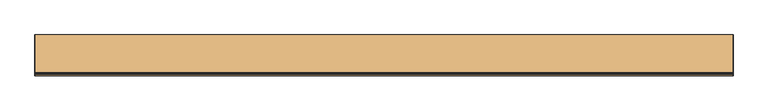
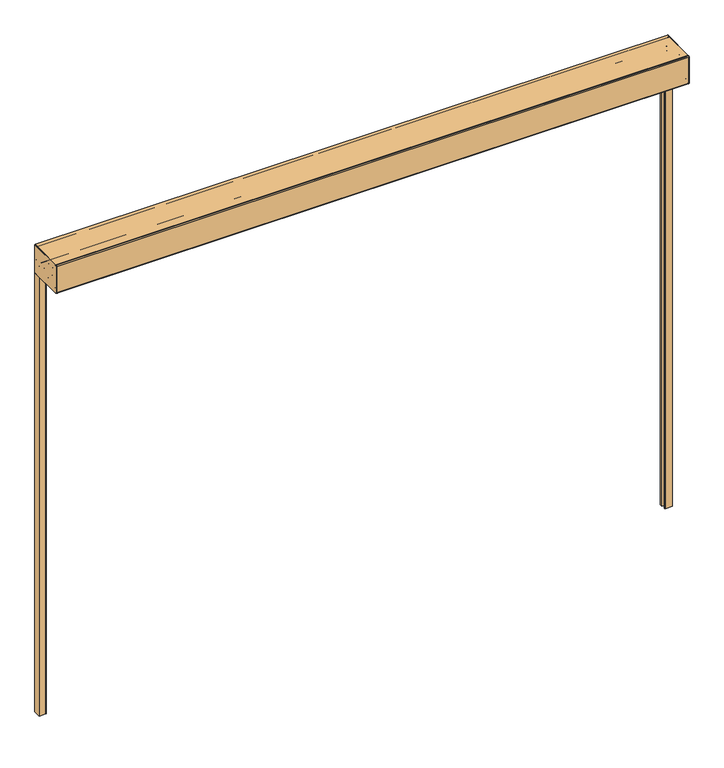
"""IFC4 building model written with IfcOpenShell, lengths in millimetres: door geometry, Otomatik Kapı-Çift Kanat : Otomatik Kapı - Çift Kanat - 150-220."""

from ifc_helpers import new_model, si_unit, point, frame, frame_2d, origin, origin_with_axes, place, context, project, spatial, polyline, circle_curve, trimmed, segment, composite_curve, outline, extrude, source, transform, mapped, element, save
from ifc_brep_helpers import plane_surface, cylinder_surface, revolved_surface, advanced_brep


def door_113a5d44(model_context):
    return source(origin(), model_context, "Body", "SolidModel", [
        advanced_brep(
        [(1494.5, -59.2542528, 2316.1817261), (1494.5, -45.0832683, 2316.1817261), (1494.5, -40.0474706, 2321.1107692), (1494.5, -40.0474706, 2324.2914876), (1494.5, 0.2446915, 2324.2914876), (1494.5, 0.2446915, 2321.2186799), (1494.5, 5.2816452, 2316.1817261), (1494.5, 13.9890898, 2316.1817261), (1494.5, 18.342812, 2313.7066015), (1494.5, 45.9985176, 2266.1506632), (1494.5, 50.8662503, 2262.4873595), (1494.5, 56.7563764, 2262.4873595), (1494.5, 61.7784339, 2267.509417), (1494.5, 61.7933302, 2276.5727956), (1494.5, 93.03701, 2276.5727956), (1494.5, 93.03701, 2265.3902264), (1494.5, 93.9651676, 2263.5834794), (1494.5, 95.0, 2261.6341872), (1494.5, 95.0, 2248.8285097), (1494.5, 94.4023169, 2246.353385), (1494.5, 78.3538909, 2218.6102552), (1494.5, 74.0001686, 2216.1339745), (1494.5, -59.2542528, 2216.1339745), (1494.5, -64.2900505, 2221.1697722), (1494.5, -64.2900505, 2311.1459284), (1494.5, -12.8153193, 2290.4871347), (1494.5, -12.8153193, 2305.6823884), (1494.5, -46.1075375, 2290.4871347), (1494.5, -46.1075375, 2305.6823884), (1494.5, -44.058999, 2251.9024734), (1494.5, -44.058999, 2266.9266302), (1494.5, 16.378666, 2251.7978536), (1494.5, 16.378666, 2267.0312501), (1494.5, -15.888127, 2223.6460529), (1494.5, -15.888127, 2238.8413066), (1494.5, 63.7563202, 2231.7558144), (1494.5, 63.7563202, 2246.7799712), (1497.5, -59.2542528, 2316.1817261), (1497.5, -64.2900505, 2311.1459284), (1497.5, -64.2900505, 2221.1697722), (1497.5, -59.2542528, 2216.1339745), (1497.5, 74.0001686, 2216.1339745), (1497.5, 78.3538909, 2218.6102552), (1497.5, 94.4023169, 2246.353385), (1497.5, 95.0, 2248.8285097), (1497.5, 95.0, 2261.6341872), (1497.5, 93.9548678, 2263.567749), (1497.5, 93.03701, 2265.3902264), (1497.5, 93.03701, 2276.5727956), (1497.5, 61.7933302, 2276.5727956), (1497.5, 61.7933302, 2267.509417), (1497.5, 56.7563764, 2262.4873595), (1497.5, 50.8662503, 2262.4873595), (1497.5, 45.9985176, 2266.1506632), (1497.5, 18.342812, 2313.7066015), (1497.5, 13.9890898, 2316.1817261), (1497.5, 5.2816452, 2316.1817261), (1497.5, 0.2446915, 2321.2186799), (1497.5, 0.2446915, 2324.2914876), (1497.5, -40.0474706, 2324.2914876), (1497.5, -40.0474706, 2321.1107692), (1497.5, -45.0832683, 2316.1817261), (1497.5, -12.8153193, 2290.4871347), (1497.5, -12.8153193, 2305.6823884), (1497.5, -46.1075375, 2290.4871347), (1497.5, -46.1075375, 2305.6823884), (1497.5, -44.058999, 2251.9024734), (1497.5, -44.058999, 2266.9266302), (1497.5, 16.378666, 2251.7978536), (1497.5, 16.378666, 2267.0312501), (1497.5, -15.888127, 2223.6460529), (1497.5, -15.888127, 2238.8413066), (1497.5, 63.7563202, 2231.7558144), (1497.5, 63.7563202, 2246.7799712)],
        [
            (0, 1),
            (1, 2, circle_curve(frame((1494.5, -45.0832683, 2321.2186799), z_axis=(1.0, 0.0, 0.0), x_axis=(0.0, 0.0, 1.0)), 5.0369538)),
            (2, 3),
            (3, 4),
            (4, 5),
            (5, 6, circle_curve(frame((1494.5, 5.2816452, 2321.2186799), z_axis=(1.0, 0.0, 0.0), x_axis=(0.0, 0.0, 1.0)), 5.0369538)),
            (6, 7),
            (7, 8, circle_curve(frame((1494.5, 14.039751, 2311.2041971), z_axis=(-1.0, 0.0, 0.0), x_axis=(0.0, 0.0, 1.0)), 4.9777868)),
            (8, 9),
            (9, 10, circle_curve(frame((1494.5, 50.8662503, 2267.5530897), z_axis=(1.0, 0.0, 0.0), x_axis=(0.0, 0.0, 1.0)), 5.0657302)),
            (10, 11),
            (11, 12, circle_curve(frame((1494.5, 56.7563764, 2267.509417), z_axis=(1.0, 0.0, 0.0), x_axis=(0.0, 0.0, 1.0)), 5.0220574)),
            (12, 13),
            (13, 14),
            (14, 15),
            (15, 16, circle_curve(frame((1494.5, 95.0917008, 2265.3039782), z_axis=(1.0, 0.0, 0.0), x_axis=(0.0, 0.0, 1.0)), 2.0565002)),
            (16, 17, circle_curve(frame((1494.5, 92.6888271, 2261.6341872), z_axis=(-1.0, 0.0, 0.0), x_axis=(0.0, 0.0, 1.0)), 2.3111729)),
            (17, 18),
            (18, 19, circle_curve(frame((1494.5, 90.5157638, 2248.6016195), z_axis=(-1.0, 0.0, 0.0), x_axis=(0.0, 0.0, 1.0)), 4.4899725)),
            (19, 20),
            (20, 21, circle_curve(frame((1494.5, 74.0600786, 2221.0940748), z_axis=(-1.0, 0.0, 0.0), x_axis=(0.0, 0.0, 1.0)), 4.9604621)),
            (21, 22),
            (22, 23, circle_curve(frame((1494.5, -59.2542528, 2221.1697722), z_axis=(-1.0, 0.0, 0.0), x_axis=(0.0, 0.0, 1.0)), 5.0357977)),
            (23, 24),
            (24, 0, circle_curve(frame((1494.5, -59.2542528, 2311.1459284), z_axis=(-1.0, 0.0, 0.0), x_axis=(0.0, 0.0, 1.0)), 5.0357977)),
            (25, 26, circle_curve(frame((1494.5, -12.8153193, 2298.0847616), z_axis=(1.0, 0.0, 0.0), x_axis=(0.0, 0.0, 1.0)), 7.5976269)),
            (26, 25, circle_curve(frame((1494.5, -12.8153193, 2298.0847616), z_axis=(1.0, 0.0, 0.0), x_axis=(0.0, 0.0, 1.0)), 7.5976269)),
            (27, 28, circle_curve(frame((1494.5, -46.1075375, 2298.0847616), z_axis=(1.0, 0.0, 0.0), x_axis=(0.0, 0.0, 1.0)), 7.5976269)),
            (28, 27, circle_curve(frame((1494.5, -46.1075375, 2298.0847616), z_axis=(1.0, 0.0, 0.0), x_axis=(0.0, 0.0, 1.0)), 7.5976269)),
            (29, 30, circle_curve(frame((1494.5, -44.058999, 2259.4145518), z_axis=(1.0, 0.0, 0.0), x_axis=(0.0, 0.0, 1.0)), 7.5120784)),
            (30, 29, circle_curve(frame((1494.5, -44.058999, 2259.4145518), z_axis=(1.0, 0.0, 0.0), x_axis=(0.0, 0.0, 1.0)), 7.5120784)),
            (31, 32, circle_curve(frame((1494.5, 16.378666, 2259.4145518), z_axis=(1.0, 0.0, 0.0), x_axis=(0.0, 0.0, 1.0)), 7.6166982)),
            (32, 31, circle_curve(frame((1494.5, 16.378666, 2259.4145518), z_axis=(1.0, 0.0, 0.0), x_axis=(0.0, 0.0, 1.0)), 7.6166982)),
            (33, 34, circle_curve(frame((1494.5, -15.888127, 2231.2436798), z_axis=(1.0, 0.0, 0.0), x_axis=(0.0, 0.0, 1.0)), 7.5976269)),
            (34, 33, circle_curve(frame((1494.5, -15.888127, 2231.2436798), z_axis=(1.0, 0.0, 0.0), x_axis=(0.0, 0.0, 1.0)), 7.5976269)),
            (35, 36, circle_curve(frame((1494.5, 63.7563202, 2239.2678928), z_axis=(1.0, 0.0, 0.0), x_axis=(0.0, 0.0, 1.0)), 7.5120784)),
            (36, 35, circle_curve(frame((1494.5, 63.7563202, 2239.2678928), z_axis=(1.0, 0.0, 0.0), x_axis=(0.0, 0.0, 1.0)), 7.5120784)),
            (37, 38, circle_curve(frame((1497.5, -59.2542528, 2311.1459284), z_axis=(1.0, 0.0, 0.0), x_axis=(0.0, 0.0, 1.0)), 5.0357977)),
            (38, 39),
            (39, 40, circle_curve(frame((1497.5, -59.2542528, 2221.1697722), z_axis=(1.0, 0.0, 0.0), x_axis=(0.0, 0.0, 1.0)), 5.0357977)),
            (40, 41),
            (41, 42, circle_curve(frame((1497.5, 74.0600786, 2221.0940748), z_axis=(1.0, 0.0, 0.0), x_axis=(0.0, 0.0, 1.0)), 4.9604621)),
            (42, 43),
            (43, 44, circle_curve(frame((1497.5, 90.5157638, 2248.6016195), z_axis=(1.0, 0.0, 0.0), x_axis=(0.0, 0.0, 1.0)), 4.4899725)),
            (44, 45),
            (45, 46, circle_curve(frame((1497.5, 92.6888271, 2261.6341872), z_axis=(1.0, 0.0, 0.0), x_axis=(0.0, 0.0, 1.0)), 2.3111729)),
            (46, 47, circle_curve(frame((1497.5, 95.0917008, 2265.3039782), z_axis=(-1.0, 0.0, 0.0), x_axis=(0.0, 0.0, 1.0)), 2.0565002)),
            (47, 48),
            (48, 49),
            (49, 50),
            (50, 51, circle_curve(frame((1497.5, 56.7563764, 2267.509417), z_axis=(-1.0, 0.0, 0.0), x_axis=(0.0, 0.0, 1.0)), 5.0220574)),
            (51, 52),
            (52, 53, circle_curve(frame((1497.5, 50.8662503, 2267.5530897), z_axis=(-1.0, 0.0, 0.0), x_axis=(0.0, 0.0, 1.0)), 5.0657302)),
            (53, 54),
            (54, 55, circle_curve(frame((1497.5, 14.039751, 2311.2041971), z_axis=(1.0, 0.0, 0.0), x_axis=(0.0, 0.0, 1.0)), 4.9777868)),
            (55, 56),
            (56, 57, circle_curve(frame((1497.5, 5.2816452, 2321.2186799), z_axis=(-1.0, 0.0, 0.0), x_axis=(0.0, 0.0, 1.0)), 5.0369538)),
            (57, 58),
            (58, 59),
            (59, 60),
            (60, 61, circle_curve(frame((1497.5, -45.0832683, 2321.2186799), z_axis=(-1.0, 0.0, 0.0), x_axis=(0.0, 0.0, 1.0)), 5.0369538)),
            (61, 37),
            (62, 63, circle_curve(frame((1497.5, -12.8153193, 2298.0847616), z_axis=(-1.0, 0.0, 0.0), x_axis=(0.0, 0.0, 1.0)), 7.5976269)),
            (63, 62, circle_curve(frame((1497.5, -12.8153193, 2298.0847616), z_axis=(-1.0, 0.0, 0.0), x_axis=(0.0, 0.0, 1.0)), 7.5976269)),
            (64, 65, circle_curve(frame((1497.5, -46.1075375, 2298.0847616), z_axis=(-1.0, 0.0, 0.0), x_axis=(0.0, 0.0, 1.0)), 7.5976269)),
            (65, 64, circle_curve(frame((1497.5, -46.1075375, 2298.0847616), z_axis=(-1.0, 0.0, 0.0), x_axis=(0.0, 0.0, 1.0)), 7.5976269)),
            (66, 67, circle_curve(frame((1497.5, -44.058999, 2259.4145518), z_axis=(-1.0, 0.0, 0.0), x_axis=(0.0, 0.0, 1.0)), 7.5120784)),
            (67, 66, circle_curve(frame((1497.5, -44.058999, 2259.4145518), z_axis=(-1.0, 0.0, 0.0), x_axis=(0.0, 0.0, 1.0)), 7.5120784)),
            (68, 69, circle_curve(frame((1497.5, 16.378666, 2259.4145518), z_axis=(-1.0, 0.0, 0.0), x_axis=(0.0, 0.0, 1.0)), 7.6166982)),
            (69, 68, circle_curve(frame((1497.5, 16.378666, 2259.4145518), z_axis=(-1.0, 0.0, 0.0), x_axis=(0.0, 0.0, 1.0)), 7.6166982)),
            (70, 71, circle_curve(frame((1497.5, -15.888127, 2231.2436798), z_axis=(-1.0, 0.0, 0.0), x_axis=(0.0, 0.0, 1.0)), 7.5976269)),
            (71, 70, circle_curve(frame((1497.5, -15.888127, 2231.2436798), z_axis=(-1.0, 0.0, 0.0), x_axis=(0.0, 0.0, 1.0)), 7.5976269)),
            (72, 73, circle_curve(frame((1497.5, 63.7563202, 2239.2678928), z_axis=(-1.0, 0.0, 0.0), x_axis=(0.0, 0.0, 1.0)), 7.5120784)),
            (73, 72, circle_curve(frame((1497.5, 63.7563202, 2239.2678928), z_axis=(-1.0, 0.0, 0.0), x_axis=(0.0, 0.0, 1.0)), 7.5120784)),
            (0, 37),
            (61, 1),
            (60, 2),
            (59, 3),
            (58, 4),
            (57, 5),
            (56, 6),
            (55, 7),
            (54, 8),
            (53, 9),
            (52, 10),
            (51, 11),
            (50, 12),
            (49, 13),
            (48, 14),
            (47, 15),
            (46, 16),
            (45, 17),
            (44, 18),
            (43, 19),
            (42, 20),
            (41, 21),
            (40, 22),
            (39, 23),
            (38, 24),
            (25, 62),
            (63, 26),
            (27, 64),
            (65, 28),
            (29, 66),
            (67, 30),
            (31, 68),
            (69, 32),
            (33, 70),
            (71, 34),
            (35, 72),
            (73, 36),
        ],
        [
            plane_surface(frame((1494.5, 95.0, 2200.0), z_axis=(-1.0, 0.0, 0.0), x_axis=(0.0, -1.0, 0.0))),
            plane_surface(frame((1497.5, 95.0, 2200.0), z_axis=(1.0, 0.0, 0.0), x_axis=(0.0, -1.0, 0.0))),
            plane_surface(frame((1494.5, -59.2542528, 2316.1817261), z_axis=(0.0, 0.0, 1.0), x_axis=(1.0, 0.0, 0.0))),
            revolved_surface(polyline([(1497.5, -45.0832683, 2326.2556337), (1494.5, -45.0832683, 2326.2556337)]), (1494.5, -45.0832683, 2321.2186799), (1.0, 0.0, 0.0)),
            plane_surface(frame((1494.5, -40.0474706, 2321.1107692), z_axis=(0.0, -1.0, 0.0), x_axis=(1.0, 0.0, 0.0))),
            plane_surface(frame((1494.5, -40.0474706, 2324.2914876), z_axis=(0.0, 0.0, 1.0), x_axis=(1.0, 0.0, 0.0))),
            plane_surface(frame((1494.5, 0.2446915, 2324.2914876), z_axis=(0.0, 1.0, 0.0), x_axis=(1.0, 0.0, 0.0))),
            revolved_surface(polyline([(1497.5, 5.2816452, 2326.2556337), (1494.5, 5.2816452, 2326.2556337)]), (1494.5, 5.2816452, 2321.2186799), (1.0, 0.0, 0.0)),
            plane_surface(frame((1494.5, 5.2816452, 2316.1817261), z_axis=(0.0, 0.0, 1.0), x_axis=(1.0, 0.0, 0.0))),
            cylinder_surface(frame((1494.5, 14.039751, 2311.2041971), z_axis=(-1.0, 0.0, 0.0), x_axis=(0.0, 0.0, 1.0)), 4.9777868),
            plane_surface(frame((1494.5, 18.342812, 2313.7066015), z_axis=(0.0, 0.8644526484288484, 0.5027142514633436), x_axis=(1.0, 0.0, 0.0))),
            revolved_surface(polyline([(1497.5, 50.8662503, 2272.6188199), (1494.5, 50.8662503, 2272.6188199)]), (1494.5, 50.8662503, 2267.5530897), (1.0, 0.0, 0.0)),
            plane_surface(frame((1494.5, 50.8662503, 2262.4873595), z_axis=(0.0, 0.0, 1.0), x_axis=(1.0, 0.0, 0.0))),
            revolved_surface(polyline([(1497.5, 56.7563764, 2272.5314744), (1494.5, 56.7563764, 2272.5314744)]), (1494.5, 56.7563764, 2267.509417), (1.0, 0.0, 0.0)),
            plane_surface(frame((1494.5, 61.7933302, 2267.509417), z_axis=(0.0, -1.0, 0.0), x_axis=(1.0, 0.0, 0.0))),
            plane_surface(frame((1494.5, 61.7933302, 2276.5727956), z_axis=(0.0, 0.0, 1.0), x_axis=(1.0, 0.0, 0.0))),
            plane_surface(frame((1494.5, 93.03701, 2276.5727956), z_axis=(0.0, 1.0, 0.0), x_axis=(1.0, 0.0, 0.0))),
            revolved_surface(polyline([(1497.5, 95.0917008, 2267.3604784), (1494.5, 95.0917008, 2267.3604784)]), (1494.5, 95.0917008, 2265.3039782), (1.0, 0.0, 0.0)),
            cylinder_surface(frame((1494.5, 92.6888271, 2261.6341872), z_axis=(-1.0, 0.0, 0.0), x_axis=(0.0, 0.0, 1.0)), 2.3111729),
            plane_surface(frame((1494.5, 95.0, 2261.6341872), z_axis=(0.0, 1.0, 0.0), x_axis=(1.0, 0.0, 0.0))),
            cylinder_surface(frame((1494.5, 90.5157638, 2248.6016195), z_axis=(-1.0, 0.0, 0.0), x_axis=(0.0, 0.0, 1.0)), 4.4899725),
            plane_surface(frame((1494.5, 94.4023169, 2246.353385), z_axis=(0.0, 0.8656073271784467, -0.5007234317814432), x_axis=(1.0, 0.0, 0.0))),
            cylinder_surface(frame((1494.5, 74.0600786, 2221.0940748), z_axis=(-1.0, 0.0, 0.0), x_axis=(0.0, 0.0, 1.0)), 4.9604621),
            plane_surface(frame((1494.5, 74.0001686, 2216.1339745), z_axis=(0.0, 0.0, -1.0), x_axis=(1.0, 0.0, 0.0))),
            cylinder_surface(frame((1494.5, -59.2542528, 2221.1697722), z_axis=(-1.0, 0.0, 0.0), x_axis=(0.0, 0.0, 1.0)), 5.0357977),
            plane_surface(frame((1494.5, -64.2900505, 2221.1697722), z_axis=(0.0, -1.0, 0.0), x_axis=(1.0, 0.0, 0.0))),
            cylinder_surface(frame((1494.5, -59.2542528, 2311.1459284), z_axis=(-1.0, 0.0, 0.0), x_axis=(0.0, 0.0, 1.0)), 5.0357977),
            revolved_surface(polyline([(1497.5, -12.8153193, 2305.6823885), (1494.5, -12.8153193, 2305.6823885)]), (1494.5, -12.8153193, 2298.0847616), (1.0, 0.0, 0.0)),
            revolved_surface(polyline([(1497.5, -46.1075375, 2305.6823885), (1494.5, -46.1075375, 2305.6823885)]), (1494.5, -46.1075375, 2298.0847616), (1.0, 0.0, 0.0)),
            revolved_surface(polyline([(1497.5, -44.058999, 2266.9266302), (1494.5, -44.058999, 2266.9266302)]), (1494.5, -44.058999, 2259.4145518), (1.0, 0.0, 0.0)),
            revolved_surface(polyline([(1497.5, 16.378666, 2267.03125), (1494.5, 16.378666, 2267.03125)]), (1494.5, 16.378666, 2259.4145518), (1.0, 0.0, 0.0)),
            revolved_surface(polyline([(1497.5, -15.888127, 2238.8413066999997), (1494.5, -15.888127, 2238.8413066999997)]), (1494.5, -15.888127, 2231.2436798), (1.0, 0.0, 0.0)),
            revolved_surface(polyline([(1497.5, 63.7563202, 2246.7799712), (1494.5, 63.7563202, 2246.7799712)]), (1494.5, 63.7563202, 2239.2678928), (1.0, 0.0, 0.0)),
        ],
        [
            (0, [[1, 2, 3, 4, 5, 6, 7, 8, 9, 10, 11, 12, 13, 14, 15, 16, 17, 18, 19, 20, 21, 22, 23, 24, 25], [26, 27], [28, 29], [30, 31], [32, 33], [34, 35], [36, 37]]),
            (1, [[38, 39, 40, 41, 42, 43, 44, 45, 46, 47, 48, 49, 50, 51, 52, 53, 54, 55, 56, 57, 58, 59, 60, 61, 62], [63, 64], [65, 66], [67, 68], [69, 70], [71, 72], [73, 74]]),
            (2, [[-1, 75, -62, 76]]),
            (3, [[-2, -76, -61, 77]]),
            (4, [[-3, -77, -60, 78]]),
            (5, [[-4, -78, -59, 79]]),
            (6, [[-5, -79, -58, 80]]),
            (7, [[-6, -80, -57, 81]]),
            (8, [[-7, -81, -56, 82]]),
            (9, [[-8, -82, -55, 83]]),
            (10, [[-9, -83, -54, 84]]),
            (11, [[-10, -84, -53, 85]]),
            (12, [[-11, -85, -52, 86]]),
            (13, [[-12, -86, -51, 87]]),
            (14, [[-13, -87, -50, 88]]),
            (15, [[-14, -88, -49, 89]]),
            (16, [[-15, -89, -48, 90]]),
            (17, [[-16, -90, -47, 91]]),
            (18, [[-17, -91, -46, 92]]),
            (19, [[-18, -92, -45, 93]]),
            (20, [[-19, -93, -44, 94]]),
            (21, [[-20, -94, -43, 95]]),
            (22, [[-21, -95, -42, 96]]),
            (23, [[-22, -96, -41, 97]]),
            (24, [[-23, -97, -40, 98]]),
            (25, [[-24, -98, -39, 99]]),
            (26, [[-25, -99, -38, -75]]),
            (27, [[-26, 100, -64, 101]]),
            (27, [[-27, -101, -63, -100]]),
            (28, [[-28, 102, -66, 103]]),
            (28, [[-29, -103, -65, -102]]),
            (29, [[-30, 104, -68, 105]]),
            (29, [[-31, -105, -67, -104]]),
            (30, [[-32, 106, -70, 107]]),
            (30, [[-33, -107, -69, -106]]),
            (31, [[-34, 108, -72, 109]]),
            (31, [[-35, -109, -71, -108]]),
            (32, [[-36, 110, -74, 111]]),
            (32, [[-37, -111, -73, -110]]),
        ],
    ),
        advanced_brep(
        [(-1494.5, 0.2446915, 2324.2914876), (-1494.5, -40.0474706, 2324.2914876), (-1494.5, -40.0474706, 2321.1107692), (-1494.5, -45.0832683, 2316.1817261), (-1494.5, -59.2542528, 2316.1817261), (-1494.5, -64.2900505, 2311.1459284), (-1494.5, -64.2900505, 2221.1697722), (-1494.5, -59.2542528, 2216.1339745), (-1494.5, 74.0001686, 2216.1339745), (-1494.5, 78.3538909, 2218.6102552), (-1494.5, 94.4023169, 2246.353385), (-1494.5, 95.0, 2248.8285097), (-1494.5, 95.0, 2261.6341872), (-1494.5, 93.9548678, 2263.567749), (-1494.5, 93.03701, 2265.3902264), (-1494.5, 93.03701, 2276.5727956), (-1494.5, 61.7933302, 2276.5727956), (-1494.5, 61.7933302, 2267.509417), (-1494.5, 56.7563764, 2262.4873595), (-1494.5, 50.8662503, 2262.4873595), (-1494.5, 45.9985176, 2266.1506632), (-1494.5, 18.342812, 2313.7066015), (-1494.5, 13.9890898, 2316.1817261), (-1494.5, 5.2816452, 2316.1817261), (-1494.5, 0.2446915, 2321.2186799), (-1494.5, 63.7563202, 2246.7799712), (-1494.5, 63.7563202, 2231.7558144), (-1494.5, 16.378666, 2267.0312501), (-1494.5, 16.378666, 2251.7978536), (-1494.5, -12.8153193, 2305.6823884), (-1494.5, -12.8153193, 2290.4871347), (-1494.5, -46.1075375, 2305.6823884), (-1494.5, -46.1075375, 2290.4871347), (-1494.5, -44.058999, 2266.9266302), (-1494.5, -44.058999, 2251.9024734), (-1494.5, -15.888127, 2238.8413066), (-1494.5, -15.888127, 2223.6460529), (-1497.5, 0.2446915, 2324.2914876), (-1497.5, 0.2446915, 2321.2186799), (-1497.5, 5.2816452, 2316.1817261), (-1497.5, 13.9890898, 2316.1817261), (-1497.5, 18.342812, 2313.7066015), (-1497.5, 45.9985176, 2266.1506632), (-1497.5, 50.8662503, 2262.4873595), (-1497.5, 56.7563764, 2262.4873595), (-1497.5, 61.7784339, 2267.509417), (-1497.5, 61.7933302, 2276.5727956), (-1497.5, 93.03701, 2276.5727956), (-1497.5, 93.03701, 2265.3902264), (-1497.5, 93.9651676, 2263.5834794), (-1497.5, 95.0, 2261.6341872), (-1497.5, 95.0, 2248.8285097), (-1497.5, 94.4023169, 2246.353385), (-1497.5, 78.3538909, 2218.6102552), (-1497.5, 74.0001686, 2216.1339745), (-1497.5, -59.2542528, 2216.1339745), (-1497.5, -64.2900505, 2221.1697722), (-1497.5, -64.2900505, 2311.1459284), (-1497.5, -59.2542528, 2316.1817261), (-1497.5, -45.0832683, 2316.1817261), (-1497.5, -40.0474706, 2321.1107692), (-1497.5, -40.0474706, 2324.2914876), (-1497.5, 63.7563202, 2246.7799712), (-1497.5, 63.7563202, 2231.7558144), (-1497.5, 16.378666, 2267.0312501), (-1497.5, 16.378666, 2251.7978536), (-1497.5, -12.8153193, 2305.6823884), (-1497.5, -12.8153193, 2290.4871347), (-1497.5, -46.1075375, 2305.6823884), (-1497.5, -46.1075375, 2290.4871347), (-1497.5, -44.058999, 2266.9266302), (-1497.5, -44.058999, 2251.9024734), (-1497.5, -15.888127, 2238.8413066), (-1497.5, -15.888127, 2223.6460529)],
        [
            (0, 1),
            (1, 2),
            (2, 3, circle_curve(frame((-1494.5, -45.0832683, 2321.2186799), z_axis=(-1.0, 0.0, 0.0), x_axis=(0.0, 0.0, -1.0)), 5.0369538)),
            (3, 4),
            (4, 5, circle_curve(frame((-1494.5, -59.2542528, 2311.1459284), z_axis=(1.0, 0.0, 0.0), x_axis=(0.0, 0.0, -1.0)), 5.0357977)),
            (5, 6),
            (6, 7, circle_curve(frame((-1494.5, -59.2542528, 2221.1697722), z_axis=(1.0, 0.0, 0.0), x_axis=(0.0, 0.0, -1.0)), 5.0357977)),
            (7, 8),
            (8, 9, circle_curve(frame((-1494.5, 74.0600786, 2221.0940748), z_axis=(1.0, 0.0, 0.0), x_axis=(0.0, 0.0, -1.0)), 4.9604621)),
            (9, 10),
            (10, 11, circle_curve(frame((-1494.5, 90.5157638, 2248.6016195), z_axis=(1.0, 0.0, 0.0), x_axis=(0.0, 0.0, -1.0)), 4.4899725)),
            (11, 12),
            (12, 13, circle_curve(frame((-1494.5, 92.6888271, 2261.6341872), z_axis=(1.0, 0.0, 0.0), x_axis=(0.0, 0.0, -1.0)), 2.3111729)),
            (13, 14, circle_curve(frame((-1494.5, 95.0917008, 2265.3039782), z_axis=(-1.0, 0.0, 0.0), x_axis=(0.0, 0.0, -1.0)), 2.0565002)),
            (14, 15),
            (15, 16),
            (16, 17),
            (17, 18, circle_curve(frame((-1494.5, 56.7563764, 2267.509417), z_axis=(-1.0, 0.0, 0.0), x_axis=(0.0, 0.0, -1.0)), 5.0220574)),
            (18, 19),
            (19, 20, circle_curve(frame((-1494.5, 50.8662503, 2267.5530897), z_axis=(-1.0, 0.0, 0.0), x_axis=(0.0, 0.0, -1.0)), 5.0657302)),
            (20, 21),
            (21, 22, circle_curve(frame((-1494.5, 14.039751, 2311.2041971), z_axis=(1.0, 0.0, 0.0), x_axis=(0.0, 0.0, -1.0)), 4.9777868)),
            (22, 23),
            (23, 24, circle_curve(frame((-1494.5, 5.2816452, 2321.2186799), z_axis=(-1.0, 0.0, 0.0), x_axis=(0.0, 0.0, -1.0)), 5.0369538)),
            (24, 0),
            (25, 26, circle_curve(frame((-1494.5, 63.7563202, 2239.2678928), z_axis=(-1.0, 0.0, 0.0), x_axis=(0.0, 0.0, -1.0)), 7.5120784)),
            (26, 25, circle_curve(frame((-1494.5, 63.7563202, 2239.2678928), z_axis=(-1.0, 0.0, 0.0), x_axis=(0.0, 0.0, -1.0)), 7.5120784)),
            (27, 28, circle_curve(frame((-1494.5, 16.378666, 2259.4145518), z_axis=(-1.0, 0.0, 0.0), x_axis=(0.0, 0.0, -1.0)), 7.6166982)),
            (28, 27, circle_curve(frame((-1494.5, 16.378666, 2259.4145518), z_axis=(-1.0, 0.0, 0.0), x_axis=(0.0, 0.0, -1.0)), 7.6166982)),
            (29, 30, circle_curve(frame((-1494.5, -12.8153193, 2298.0847616), z_axis=(-1.0, 0.0, 0.0), x_axis=(0.0, 0.0, -1.0)), 7.5976269)),
            (30, 29, circle_curve(frame((-1494.5, -12.8153193, 2298.0847616), z_axis=(-1.0, 0.0, 0.0), x_axis=(0.0, 0.0, -1.0)), 7.5976269)),
            (31, 32, circle_curve(frame((-1494.5, -46.1075375, 2298.0847616), z_axis=(-1.0, 0.0, 0.0), x_axis=(0.0, 0.0, -1.0)), 7.5976269)),
            (32, 31, circle_curve(frame((-1494.5, -46.1075375, 2298.0847616), z_axis=(-1.0, 0.0, 0.0), x_axis=(0.0, 0.0, -1.0)), 7.5976269)),
            (33, 34, circle_curve(frame((-1494.5, -44.058999, 2259.4145518), z_axis=(-1.0, 0.0, 0.0), x_axis=(0.0, 0.0, -1.0)), 7.5120784)),
            (34, 33, circle_curve(frame((-1494.5, -44.058999, 2259.4145518), z_axis=(-1.0, 0.0, 0.0), x_axis=(0.0, 0.0, -1.0)), 7.5120784)),
            (35, 36, circle_curve(frame((-1494.5, -15.888127, 2231.2436798), z_axis=(-1.0, 0.0, 0.0), x_axis=(0.0, 0.0, -1.0)), 7.5976269)),
            (36, 35, circle_curve(frame((-1494.5, -15.888127, 2231.2436798), z_axis=(-1.0, 0.0, 0.0), x_axis=(0.0, 0.0, -1.0)), 7.5976269)),
            (37, 38),
            (38, 39, circle_curve(frame((-1497.5, 5.2816452, 2321.2186799), z_axis=(1.0, 0.0, 0.0), x_axis=(0.0, 0.0, -1.0)), 5.0369538)),
            (39, 40),
            (40, 41, circle_curve(frame((-1497.5, 14.039751, 2311.2041971), z_axis=(-1.0, 0.0, 0.0), x_axis=(0.0, 0.0, -1.0)), 4.9777868)),
            (41, 42),
            (42, 43, circle_curve(frame((-1497.5, 50.8662503, 2267.5530897), z_axis=(1.0, 0.0, 0.0), x_axis=(0.0, 0.0, -1.0)), 5.0657302)),
            (43, 44),
            (44, 45, circle_curve(frame((-1497.5, 56.7563764, 2267.509417), z_axis=(1.0, 0.0, 0.0), x_axis=(0.0, 0.0, -1.0)), 5.0220574)),
            (45, 46),
            (46, 47),
            (47, 48),
            (48, 49, circle_curve(frame((-1497.5, 95.0917008, 2265.3039782), z_axis=(1.0, 0.0, 0.0), x_axis=(0.0, 0.0, -1.0)), 2.0565002)),
            (49, 50, circle_curve(frame((-1497.5, 92.6888271, 2261.6341872), z_axis=(-1.0, 0.0, 0.0), x_axis=(0.0, 0.0, -1.0)), 2.3111729)),
            (50, 51),
            (51, 52, circle_curve(frame((-1497.5, 90.5157638, 2248.6016195), z_axis=(-1.0, 0.0, 0.0), x_axis=(0.0, 0.0, -1.0)), 4.4899725)),
            (52, 53),
            (53, 54, circle_curve(frame((-1497.5, 74.0600786, 2221.0940748), z_axis=(-1.0, 0.0, 0.0), x_axis=(0.0, 0.0, -1.0)), 4.9604621)),
            (54, 55),
            (55, 56, circle_curve(frame((-1497.5, -59.2542528, 2221.1697722), z_axis=(-1.0, 0.0, 0.0), x_axis=(0.0, 0.0, -1.0)), 5.0357977)),
            (56, 57),
            (57, 58, circle_curve(frame((-1497.5, -59.2542528, 2311.1459284), z_axis=(-1.0, 0.0, 0.0), x_axis=(0.0, 0.0, -1.0)), 5.0357977)),
            (58, 59),
            (59, 60, circle_curve(frame((-1497.5, -45.0832683, 2321.2186799), z_axis=(1.0, 0.0, 0.0), x_axis=(0.0, 0.0, -1.0)), 5.0369538)),
            (60, 61),
            (61, 37),
            (62, 63, circle_curve(frame((-1497.5, 63.7563202, 2239.2678928), z_axis=(1.0, 0.0, 0.0), x_axis=(0.0, 0.0, -1.0)), 7.5120784)),
            (63, 62, circle_curve(frame((-1497.5, 63.7563202, 2239.2678928), z_axis=(1.0, 0.0, 0.0), x_axis=(0.0, 0.0, -1.0)), 7.5120784)),
            (64, 65, circle_curve(frame((-1497.5, 16.378666, 2259.4145518), z_axis=(1.0, 0.0, 0.0), x_axis=(0.0, 0.0, -1.0)), 7.6166982)),
            (65, 64, circle_curve(frame((-1497.5, 16.378666, 2259.4145518), z_axis=(1.0, 0.0, 0.0), x_axis=(0.0, 0.0, -1.0)), 7.6166982)),
            (66, 67, circle_curve(frame((-1497.5, -12.8153193, 2298.0847616), z_axis=(1.0, 0.0, 0.0), x_axis=(0.0, 0.0, -1.0)), 7.5976269)),
            (67, 66, circle_curve(frame((-1497.5, -12.8153193, 2298.0847616), z_axis=(1.0, 0.0, 0.0), x_axis=(0.0, 0.0, -1.0)), 7.5976269)),
            (68, 69, circle_curve(frame((-1497.5, -46.1075375, 2298.0847616), z_axis=(1.0, 0.0, 0.0), x_axis=(0.0, 0.0, -1.0)), 7.5976269)),
            (69, 68, circle_curve(frame((-1497.5, -46.1075375, 2298.0847616), z_axis=(1.0, 0.0, 0.0), x_axis=(0.0, 0.0, -1.0)), 7.5976269)),
            (70, 71, circle_curve(frame((-1497.5, -44.058999, 2259.4145518), z_axis=(1.0, 0.0, 0.0), x_axis=(0.0, 0.0, -1.0)), 7.5120784)),
            (71, 70, circle_curve(frame((-1497.5, -44.058999, 2259.4145518), z_axis=(1.0, 0.0, 0.0), x_axis=(0.0, 0.0, -1.0)), 7.5120784)),
            (72, 73, circle_curve(frame((-1497.5, -15.888127, 2231.2436798), z_axis=(1.0, 0.0, 0.0), x_axis=(0.0, 0.0, -1.0)), 7.5976269)),
            (73, 72, circle_curve(frame((-1497.5, -15.888127, 2231.2436798), z_axis=(1.0, 0.0, 0.0), x_axis=(0.0, 0.0, -1.0)), 7.5976269)),
            (0, 37),
            (61, 1),
            (60, 2),
            (59, 3),
            (58, 4),
            (57, 5),
            (56, 6),
            (55, 7),
            (54, 8),
            (53, 9),
            (52, 10),
            (51, 11),
            (50, 12),
            (49, 13),
            (48, 14),
            (47, 15),
            (46, 16),
            (45, 17),
            (44, 18),
            (43, 19),
            (42, 20),
            (41, 21),
            (40, 22),
            (39, 23),
            (38, 24),
            (25, 62),
            (63, 26),
            (27, 64),
            (65, 28),
            (29, 66),
            (67, 30),
            (31, 68),
            (69, 32),
            (33, 70),
            (71, 34),
            (35, 72),
            (73, 36),
        ],
        [
            plane_surface(frame((-1494.5, 95.0, 2199.9969475), z_axis=(1.0, 0.0, 0.0), x_axis=(0.0, -1.0, 0.0))),
            plane_surface(frame((-1497.5, 95.0, 2199.9969475), z_axis=(-1.0, 0.0, 0.0), x_axis=(0.0, -1.0, 0.0))),
            plane_surface(frame((-1494.5, 0.2446915, 2324.2914876), z_axis=(0.0, 0.0, 1.0), x_axis=(-1.0, 0.0, 0.0))),
            plane_surface(frame((-1494.5, -40.0474706, 2324.2914876), z_axis=(0.0, -1.0, 0.0), x_axis=(-1.0, 0.0, 0.0))),
            revolved_surface(polyline([(-1497.5, -45.0832683, 2316.1817261), (-1494.5, -45.0832683, 2316.1817261)]), (-1494.5, -45.0832683, 2321.2186799), (-1.0, 0.0, 0.0)),
            plane_surface(frame((-1494.5, -45.0832683, 2316.1817261), z_axis=(0.0, 0.0, 1.0), x_axis=(-1.0, 0.0, 0.0))),
            cylinder_surface(frame((-1494.5, -59.2542528, 2311.1459284), z_axis=(1.0, 0.0, 0.0), x_axis=(0.0, 0.0, -1.0)), 5.0357977),
            plane_surface(frame((-1494.5, -64.2900505, 2311.1459284), z_axis=(0.0, -1.0, 0.0), x_axis=(-1.0, 0.0, 0.0))),
            cylinder_surface(frame((-1494.5, -59.2542528, 2221.1697722), z_axis=(1.0, 0.0, 0.0), x_axis=(0.0, 0.0, -1.0)), 5.0357977),
            plane_surface(frame((-1494.5, -59.2542528, 2216.1339745), z_axis=(0.0, 0.0, -1.0), x_axis=(-1.0, 0.0, 0.0))),
            cylinder_surface(frame((-1494.5, 74.0600786, 2221.0940748), z_axis=(1.0, 0.0, 0.0), x_axis=(0.0, 0.0, -1.0)), 4.9604621),
            plane_surface(frame((-1494.5, 78.3538909, 2218.6102552), z_axis=(0.0, 0.8656073271784469, -0.5007234317814427), x_axis=(-1.0, 0.0, 0.0))),
            cylinder_surface(frame((-1494.5, 90.5157638, 2248.6016195), z_axis=(1.0, 0.0, 0.0), x_axis=(0.0, 0.0, -1.0)), 4.4899725),
            plane_surface(frame((-1494.5, 95.0, 2248.8285097), z_axis=(0.0, 1.0, 0.0), x_axis=(-1.0, 0.0, 0.0))),
            cylinder_surface(frame((-1494.5, 92.6888271, 2261.6341872), z_axis=(1.0, 0.0, 0.0), x_axis=(0.0, 0.0, -1.0)), 2.3111729),
            revolved_surface(polyline([(-1497.5, 95.0917008, 2263.2474780000002), (-1494.5, 95.0917008, 2263.2474780000002)]), (-1494.5, 95.0917008, 2265.3039782), (-1.0, 0.0, 0.0)),
            plane_surface(frame((-1494.5, 93.03701, 2265.3902264), z_axis=(0.0, 1.0, 0.0), x_axis=(-1.0, 0.0, 0.0))),
            plane_surface(frame((-1494.5, 93.03701, 2276.5727956), z_axis=(0.0, 0.0, 1.0), x_axis=(-1.0, 0.0, 0.0))),
            plane_surface(frame((-1494.5, 61.7933302, 2276.5727956), z_axis=(0.0, -1.0, 0.0), x_axis=(-1.0, 0.0, 0.0))),
            revolved_surface(polyline([(-1497.5, 56.7563764, 2262.4873596), (-1494.5, 56.7563764, 2262.4873596)]), (-1494.5, 56.7563764, 2267.509417), (-1.0, 0.0, 0.0)),
            plane_surface(frame((-1494.5, 56.7563764, 2262.4873595), z_axis=(0.0, 0.0, 1.0), x_axis=(-1.0, 0.0, 0.0))),
            revolved_surface(polyline([(-1497.5, 50.8662503, 2262.4873595), (-1494.5, 50.8662503, 2262.4873595)]), (-1494.5, 50.8662503, 2267.5530897), (-1.0, 0.0, 0.0)),
            plane_surface(frame((-1494.5, 45.9985176, 2266.1506632), z_axis=(0.0, 0.8644526484288326, 0.5027142514633708), x_axis=(-1.0, 0.0, 0.0))),
            cylinder_surface(frame((-1494.5, 14.039751, 2311.2041971), z_axis=(1.0, 0.0, 0.0), x_axis=(0.0, 0.0, -1.0)), 4.9777868),
            plane_surface(frame((-1494.5, 13.9890898, 2316.1817261), z_axis=(0.0, 0.0, 1.0), x_axis=(-1.0, 0.0, 0.0))),
            revolved_surface(polyline([(-1497.5, 5.2816452, 2316.1817261), (-1494.5, 5.2816452, 2316.1817261)]), (-1494.5, 5.2816452, 2321.2186799), (-1.0, 0.0, 0.0)),
            plane_surface(frame((-1494.5, 0.2446915, 2321.2186799), z_axis=(0.0, 1.0, 0.0), x_axis=(-1.0, 0.0, 0.0))),
            revolved_surface(polyline([(-1497.5, 63.7563202, 2231.7558144), (-1494.5, 63.7563202, 2231.7558144)]), (-1494.5, 63.7563202, 2239.2678928), (-1.0, 0.0, 0.0)),
            revolved_surface(polyline([(-1497.5, 16.378666, 2251.7978536), (-1494.5, 16.378666, 2251.7978536)]), (-1494.5, 16.378666, 2259.4145518), (-1.0, 0.0, 0.0)),
            revolved_surface(polyline([(-1497.5, -12.8153193, 2290.4871347000003), (-1494.5, -12.8153193, 2290.4871347000003)]), (-1494.5, -12.8153193, 2298.0847616), (-1.0, 0.0, 0.0)),
            revolved_surface(polyline([(-1497.5, -46.1075375, 2290.4871347000003), (-1494.5, -46.1075375, 2290.4871347000003)]), (-1494.5, -46.1075375, 2298.0847616), (-1.0, 0.0, 0.0)),
            revolved_surface(polyline([(-1497.5, -44.058999, 2251.9024734), (-1494.5, -44.058999, 2251.9024734)]), (-1494.5, -44.058999, 2259.4145518), (-1.0, 0.0, 0.0)),
            revolved_surface(polyline([(-1497.5, -15.888127, 2223.6460529), (-1494.5, -15.888127, 2223.6460529)]), (-1494.5, -15.888127, 2231.2436798), (-1.0, 0.0, 0.0)),
        ],
        [
            (0, [[1, 2, 3, 4, 5, 6, 7, 8, 9, 10, 11, 12, 13, 14, 15, 16, 17, 18, 19, 20, 21, 22, 23, 24, 25], [26, 27], [28, 29], [30, 31], [32, 33], [34, 35], [36, 37]]),
            (1, [[38, 39, 40, 41, 42, 43, 44, 45, 46, 47, 48, 49, 50, 51, 52, 53, 54, 55, 56, 57, 58, 59, 60, 61, 62], [63, 64], [65, 66], [67, 68], [69, 70], [71, 72], [73, 74]]),
            (2, [[-1, 75, -62, 76]]),
            (3, [[-2, -76, -61, 77]]),
            (4, [[-3, -77, -60, 78]]),
            (5, [[-4, -78, -59, 79]]),
            (6, [[-5, -79, -58, 80]]),
            (7, [[-6, -80, -57, 81]]),
            (8, [[-7, -81, -56, 82]]),
            (9, [[-8, -82, -55, 83]]),
            (10, [[-9, -83, -54, 84]]),
            (11, [[-10, -84, -53, 85]]),
            (12, [[-11, -85, -52, 86]]),
            (13, [[-12, -86, -51, 87]]),
            (14, [[-13, -87, -50, 88]]),
            (15, [[-14, -88, -49, 89]]),
            (16, [[-15, -89, -48, 90]]),
            (17, [[-16, -90, -47, 91]]),
            (18, [[-17, -91, -46, 92]]),
            (19, [[-18, -92, -45, 93]]),
            (20, [[-19, -93, -44, 94]]),
            (21, [[-20, -94, -43, 95]]),
            (22, [[-21, -95, -42, 96]]),
            (23, [[-22, -96, -41, 97]]),
            (24, [[-23, -97, -40, 98]]),
            (25, [[-24, -98, -39, 99]]),
            (26, [[-25, -99, -38, -75]]),
            (27, [[-26, 100, -64, 101]]),
            (27, [[-27, -101, -63, -100]]),
            (28, [[-28, 102, -66, 103]]),
            (28, [[-29, -103, -65, -102]]),
            (29, [[-30, 104, -68, 105]]),
            (29, [[-31, -105, -67, -104]]),
            (30, [[-32, 106, -70, 107]]),
            (30, [[-33, -107, -69, -106]]),
            (31, [[-34, 108, -72, 109]]),
            (31, [[-35, -109, -71, -108]]),
            (32, [[-36, 110, -74, 111]]),
            (32, [[-37, -111, -73, -110]]),
        ],
    ),
        extrude(outline(composite_curve([segment(polyline([(-71.5000025, 2340.0002021), (95.0, 2339.9997337), (95.0, 2275.9993507), (93.5000005, 2275.9993507), (93.4999983, 2284.1994972)]), True, "CONTINUOUS"), segment(trimmed(circle_curve(frame_2d((92.4999983, 2284.1994972)), 1.0), [point((93.4999983, 2284.1994972))], [point((92.4999996, 2285.1994972))], True, "CARTESIAN"), True, "CONTINUOUS"), segment(polyline([(92.4999996, 2285.1994972), (81.4999982, 2285.1995108), (81.4999995, 2279.9993507), (70.6996729, 2279.9993507), (70.6996729, 2277.9993047), (67.2996636, 2277.9993047), (67.2996602, 2275.9993045), (47.9996989, 2275.9993507)]), True, "CONTINUOUS"), segment(trimmed(circle_curve(frame_2d((47.9996989, 2277.9993508)), 2.0), [point((47.9996989, 2275.9993507))], [point((45.9996989, 2277.9993508))], False, "CARTESIAN"), True, "CONTINUOUS"), segment(polyline([(45.9996989, 2277.9993508), (45.9996989, 2281.7851316)]), True, "CONTINUOUS"), segment(trimmed(circle_curve(frame_2d((55.0245268, 2262.7091902)), 21.1030581), [point((45.9996989, 2281.7851316))], [point((63.8244595, 2281.8899161))], False, "CARTESIAN"), True, "CONTINUOUS"), segment(polyline([(63.8244595, 2281.8899161), (64.2993601, 2281.249351), (65.2996481, 2281.249351)]), True, "CONTINUOUS"), segment(trimmed(circle_curve(frame_2d((65.2996481, 2282.2493509)), 1.0), [point((65.2996481, 2281.249351))], [point((66.2996481, 2282.2493509))], True, "CARTESIAN"), True, "CONTINUOUS"), segment(polyline([(66.2996481, 2282.2493509), (66.2996481, 2287.7993514)]), True, "CONTINUOUS"), segment(trimmed(circle_curve(frame_2d((71.2996483, 2287.7993512)), 5.0), [point((66.2996481, 2287.7993514))], [point((71.2996483, 2292.7993512))], False, "CARTESIAN"), True, "CONTINUOUS"), segment(polyline([(71.2996483, 2292.7993512), (74.4162813, 2292.7993512), (84.1196152, 2290.1993508), (88.0, 2290.1993508)]), True, "CONTINUOUS"), segment(trimmed(circle_curve(frame_2d((88.0, 2292.1993508)), 2.0), [point((88.0, 2290.1993508))], [point((90.0, 2292.1993508))], True, "CARTESIAN"), True, "CONTINUOUS"), segment(polyline([(90.0, 2292.1993508), (90.0, 2319.2557558), (84.0000326, 2322.0535694), (84.0000067, 2334.0001367)]), True, "CONTINUOUS"), segment(trimmed(circle_curve(frame_2d((82.0000067, 2334.0001324)), 2.0), [point((84.0000067, 2334.0001367))], [point((82.000002, 2336.0001324))], True, "CARTESIAN"), True, "CONTINUOUS"), segment(polyline([(82.000002, 2336.0001324), (77.5000022, 2336.0001218), (65.7923175, 2336.5001575), (-59.9320146, 2336.5000914), (-58.5859905, 2331.476655)]), True, "CONTINUOUS"), segment(trimmed(circle_curve(frame_2d((-61.4837682, 2330.7001988)), 3.0), [point((-58.5859905, 2331.476655))], [point((-61.4837692, 2327.7001988))], False, "CARTESIAN"), True, "CONTINUOUS"), segment(polyline([(-61.4837692, 2327.7001988), (-68.9997533, 2327.7002012), (-68.9997533, 2325.7002021), (-72.5800177, 2325.7002021)]), True, "CONTINUOUS"), segment(trimmed(circle_curve(frame_2d((-74.0497523, 2326.0000026)), 1.5), [point((-72.5800177, 2325.7002021))], [point((-74.0497523, 2324.5000026))], False, "CARTESIAN"), True, "CONTINUOUS"), segment(polyline([(-74.0497523, 2324.5000026), (-78.1997522, 2324.5000026), (-78.1997522, 2205.3000002)]), True, "CONTINUOUS"), segment(trimmed(circle_curve(frame_2d((-74.6997523, 2205.3000002)), 3.5), [point((-78.1997522, 2205.3000002))], [point((-76.5025277, 2202.3))], True, "CARTESIAN"), True, "CONTINUOUS"), segment(polyline([(-76.5025277, 2202.3), (-4.2769412, 2202.3), (-2.9490356, 2200.0), (-74.9997523, 2200.0)]), True, "CONTINUOUS"), segment(trimmed(circle_curve(frame_2d((-74.9997523, 2205.0000002)), 5.0), [point((-74.9997523, 2200.0))], [point((-79.9997523, 2205.0000002))], False, "CARTESIAN"), True, "CONTINUOUS"), segment(polyline([(-79.9997523, 2205.0000002), (-79.9997523, 2335.0000002)]), True, "CONTINUOUS"), segment(trimmed(circle_curve(frame_2d((-74.9997523, 2335.0000002)), 5.0), [point((-79.9997523, 2335.0000002))], [point((-77.2497337, 2339.4651523))], False, "CARTESIAN"), True, "CONTINUOUS"), segment(polyline([(-77.2497337, 2339.4651523), (-77.2497337, 2337.6809671)]), True, "CONTINUOUS"), segment(trimmed(circle_curve(frame_2d((-74.9997523, 2335.0000002)), 3.5), [point((-77.2497337, 2337.6809671))], [point((-78.4997523, 2335.0000002))], True, "CARTESIAN"), True, "CONTINUOUS"), segment(polyline([(-78.4997523, 2335.0000002), (-78.4997523, 2326.0000026), (-74.0497523, 2326.0000026), (-74.0497523, 2334.7000026)]), True, "CONTINUOUS"), segment(trimmed(circle_curve(frame_2d((-73.0497523, 2334.7000026)), 1.0), [point((-74.0497523, 2334.7000026))], [point((-73.0497523, 2335.7000026))], False, "CARTESIAN"), True, "CONTINUOUS"), segment(polyline([(-73.0497523, 2335.7000026), (-67.9497523, 2335.7000026)]), True, "CONTINUOUS"), segment(trimmed(circle_curve(frame_2d((-67.9497523, 2334.7000026)), 1.0), [point((-67.9497523, 2335.7000026))], [point((-66.9497523, 2334.7000026))], False, "CARTESIAN"), True, "CONTINUOUS"), segment(polyline([(-66.9497523, 2334.7000026), (-66.9497523, 2329.7002005), (-61.4400224, 2329.7001988)]), True, "CONTINUOUS"), segment(trimmed(circle_curve(frame_2d((-61.4400221, 2330.7001988)), 1.0), [point((-61.4400224, 2329.7001988))], [point((-60.4740962, 2330.9590176))], True, "CARTESIAN"), True, "CONTINUOUS"), segment(polyline([(-60.4740962, 2330.9590176), (-62.2000034, 2337.4001991), (-67.1397217, 2337.4002006)]), True, "CONTINUOUS"), segment(trimmed(circle_curve(frame_2d((-67.1397209, 2339.9002006)), 2.5), [point((-67.1397217, 2337.4002006))], [point((-68.3503724, 2337.7128911))], False, "CARTESIAN"), True, "CONTINUOUS"), segment(trimmed(circle_curve(frame_2d((-71.4015985, 2332.2001768)), 6.3007936), [point((-68.3503724, 2337.7128911))], [point((-71.5000029, 2338.5002019))], True, "CARTESIAN"), True, "CONTINUOUS"), segment(polyline([(-71.5000029, 2338.5002019), (-71.5000025, 2340.0002021)]), True, "CONTINUOUS")], self_intersect=False)), frame((-1497.5, 0.0, 0.0), z_axis=(1.0, 0.0, 0.0), x_axis=(0.0, 1.0, 0.0)), (0.0, 0.0, 1.0), 2995.0),
        extrude(outline(composite_curve([segment(polyline([(-75.0505182, 2339.9997448), (95.0, 2339.9997448), (95.0, 2200.0), (-75.0, 2200.0)]), True, "CONTINUOUS"), segment(trimmed(circle_curve(frame_2d((-75.0, 2205.0)), 5.0), [point((-75.0, 2200.0))], [point((-80.0, 2205.0))], False, "CARTESIAN"), True, "CONTINUOUS"), segment(polyline([(-80.0, 2205.0), (-80.0, 2335.0)]), True, "CONTINUOUS"), segment(trimmed(circle_curve(frame_2d((-75.0, 2335.0)), 5.0), [point((-80.0, 2335.0))], [point((-75.0505182, 2339.9997448))], False, "CARTESIAN"), True, "CONTINUOUS")], self_intersect=False)), frame((1497.5, 0.0, 0.0), z_axis=(1.0, 0.0, 0.0), x_axis=(0.0, 1.0, 0.0)), (0.0, 0.0, 1.0), 2.5),
        extrude(outline(composite_curve([segment(polyline([(-75.0505182, 2339.9997448), (95.0, 2339.9997448), (95.0, 2200.0), (-75.0, 2200.0)]), True, "CONTINUOUS"), segment(trimmed(circle_curve(frame_2d((-75.0, 2205.0)), 5.0), [point((-75.0, 2200.0))], [point((-80.0, 2205.0))], False, "CARTESIAN"), True, "CONTINUOUS"), segment(polyline([(-80.0, 2205.0), (-80.0, 2335.0)]), True, "CONTINUOUS"), segment(trimmed(circle_curve(frame_2d((-75.0, 2335.0)), 5.0), [point((-80.0, 2335.0))], [point((-75.0505182, 2339.9997448))], False, "CARTESIAN"), True, "CONTINUOUS")], self_intersect=False)), frame((-1500.0, 0.0, 0.0), z_axis=(1.0, 0.0, 0.0), x_axis=(0.0, 1.0, 0.0)), (0.0, 0.0, 1.0), 2.5),
        extrude(outline(polyline([(1465.0015, 95.0), (1500.0, 95.0), (1500.0, 60.0), (1468.4641016, 60.0), (1465.8113687, 61.5315561), (1465.8113687, 62.5), (1480.0, 62.5), (1480.0, 82.5), (1465.0015, 82.5), (1465.0015, 95.0)])), origin_with_axes(), (0.0, 0.0, 1.0), 2200.0),
        extrude(outline(polyline([(-1500.0, 95.0), (-1465.0015, 95.0), (-1465.0015, 82.5), (-1480.0, 82.5), (-1480.0, 62.5), (-1465.4439986, 62.5), (-1465.4439986, 61.6472183), (-1468.3119176, 59.9914245), (-1500.0, 59.9914245), (-1500.0, 95.0)])), origin_with_axes(), (0.0, 0.0, 1.0), 2200.0),
    ])


if __name__ == "__main__":
    model = new_model("IFC4")
    model_context = context("Model", 3, world=origin())
    ifc_project = project(units=[si_unit("LENGTHUNIT", "METRE", prefix="MILLI")], contexts=[model_context])
    site = spatial("IfcSite", under=ifc_project)
    building = spatial("IfcBuilding", under=site)
    placement = place(None, origin())
    door_shape = door_113a5d44(model_context)
    element("IfcDoor", 1, ObjectType="Otomatik Kapı-Çift Kanat : Otomatik Kapı - Çift Kanat - 150-220", at=placement, inside=building, context=model_context, shape_type="MappedRepresentation", body=[
        mapped(door_shape, transform((0.0, 0.0, 0.0), x_axis=(1.0, 0.0, 0.0), y_axis=(0.0, 1.0, 0.0), z_axis=(0.0, 0.0, 1.0))),
    ])
    save(model, "model.ifc")

# Revit data of these elements
# Type "Otomatik Kapı-Çift Kanat : Otomatik Kapı - Çift Kanat - 150-220"
#   Type Mark = "47"
#   Uniformat II Description = "Exterior Doors"
#   Uniformat II Code = "B2030"
#   Uniclass 2015 Name = "Sliding doorset systems"
#   Uniclass 2015 Code = "Ss_25_30_20_77"
#   Uniclass 2.0 Description = "Sliding Doorset Systems"
#   Uniclass 2.0 Code = "SS-25-30-20-77"
#   Uniclass 1.4 Description = "Doors"
#   Uniclass 1.4 Code = "L411"
#   UNSPSC Code = "30171510"
#   Technical description = "https://media.gilgendoorsystems.com/download/NcPWaystFgYr"
#   QR code = "https://bimobject.com/gilgen/product/sliding_door_psa_bi-parting_withsidepanels_inwall"
#   Product url = "https://www.gilgendoorsystems.com/en/products-and-systems/automatic-door-systems/sliding-doors/sliding-door-design-slim-frame"
#   Product name = "Automatic Sliding Door (slim frame) - Bi-parting - With side panels - In wall - SL/PSA"
#   Product group = "Automatic Sliding Doors"
#   Product family = "Automatic Sliding Doors"
#   Product data url = "https://bimobject.com/gilgen/product/sliding_door_psa_bi-parting_withsidepanels_inwall"
#   Product certification = "https://www.gilgendoorsystems.com/en/download-centre/tuev-certificates"
#   Product SKU = "Sliding_Door_PSA_Bi-parting_WithSidePanels_Inwall"
#   Product Guid = "bd2c60fb-bb7b-44f3-83a2-de894a5f6ca4"
#   OmniClass Description = "Doors"
#   OmniClass Code = "23-17 11 00"
#   Note = "230V/13A Connector socket needed, the operator also needs a voltage-free contacts for opening commande or switching between program functions"
#   NBS Reference Description = "Sliding Doorset Systems"
#   NBS Reference Code = "25-30-20-77"
#   Model = "SL PSA"
#   Material secondary = "Glass"
#   Material main = "Aluminium"
#   Masterformat 2014 Description = "Sliding Aluminum-Framed Glass Doors"
#   Masterformat 2014 Code = "08 32 13"
#   Manufacturer name = "Gilgen"
#   Manufacturer country = "Switzerland"
#   Manufacturer = "Gilgen"
#   Keynote = "08000"
#   Installation instructions = "https://media.gilgendoorsystems.com/product/sl#"
#   IFC Classification = "Door"
#   Design country = "Switzerland"
#   Date of publishing = "08.01.2020 00:00:00"
#   Colours Note = "All colours available"
#   Bottom Rail Note 2 [instance default] = "For the Drained continuous guide rail There must be flexible tubes on site to take out water (Slope < 1.5 %). The flexible tube connection is thread ½, and a EPDM foil or liquid synthetic material outside and a Air- and vapor-tight foil inside (on site)"
#   Bottom Rail Note [instance default] = "For drained and heated rails a cable from the header to the bottom rail in a M25 pipe is needed"
#   BIMobject category = "Sliding"
#   Assembly Code = "B2030100"
#   Analytic Construction = "<None>"
#   Standard Profile [instance default] = 0.00 cm
#   Rough Width = 300.00 cm
#   Rough Height [instance default] = 234.00 cm
#   Post Width = 150.84 cm
#   Pocket screen width R = 78.82 cm
#   Pocket screen width L = 78.82 cm
#   Pocket screen height [instance default] = 222.50 cm
#   Openning distance [instance default] = 3.09 cm
#   Opening Width LB = 150.00 cm
#   Opening Width Control = 150.00 cm
#   Opening Height LH = 220.00 cm
#   Moving leaf width = 75.42 cm
#   Moving leaf height [instance default] = 224.10 cm
#   Inset [instance default] = 0.00 cm
#   Header width = 299.50 cm
#   Header offset right CR = 0.00 cm
#   Header offset left CL = 0.00 cm
#   Header height [instance default] = 14.00 cm
#   Header depth [instance default] = 22.50 cm
#   Header Right Control = 0.00 cm
#   Header Left Control = 0.00 cm
#   Gap above header control [instance default] = 0.00 cm
#   Gap above header OH = 0.00 cm
#   Gap = 0.00 cm
#   Height = 220.00 cm
#   Width = 300.00 cm
#   Fixed leaf height [instance default] = 223.20 cm
#   Fixed leaf R width = 75.42 cm
#   Fixed leaf L width = 75.42 cm
#   CR max = 300.00 cm
#   CL max = 300.00 cm
#   Standard [instance default] = no
#   Side plate [instance default] = no
#   Side cap [instance default] = yes
#   Rail 4 [instance default] = no
#   Rail 3 [instance default] = no
#   Rail 2 [instance default] = no
#   Rail 1 [instance default] = no
#   Pocket screen [instance default] = yes
#   Open [instance default] = no
#   Heated [instance default] = no
#   Fixed point [instance default] = yes
#   Edition number = 1
#   Dimensions overconstraint = no
#   Connector [instance default] = no
#   Closing Profile [instance default] = yes
#   Mounting Option [instance default] = element 451667
#   Mounting G = element 451673
#   Mounting F = element 451672
#   Mounting E = element 451671
#   Mounting D = element 451670
#   Mounting C = element 451669
#   Mounting B = element 451668
#   Mounting A = element 451667
#   Header Option [instance default] = element 451680
#   Header 2 = element 451680
#   Header 1 = element 451679
#   Guide 5 = element 451678
#   Guide 4 = element 451674
#   Guide 3 = element 451677
#   Guide 2 = element 451676
#   Guide 1 = element 451675
#   Frame material = Finish_Gilgen_Aluminium
#   Bottom Guide Rail [instance default] = element 451674
#   Function = (empty or 0)
#   Wall Closure = (empty or 0)
# Element 1 (IfcDoor, "Otomatik Kapı-Çift Kanat : Otomatik Kapı - Çift Kanat - 150-220")
#   Materials on its faces: "Finish_Gilgen_Aluminium", "Glass", "Rubber, Natural", "Plastic, Opaque Black"
# Materials
#   "Finish_Gilgen_Aluminium": class "Metal", colour RGB 120 120 120, transparency 0, Description = "Aluminium", Cost = 0
#   "Glass": class "Glass", colour RGB 0 128 192, transparency 0.9, Description = "Soda Lime Glass", Cost = 0
#   "Rubber, Natural": class "Plastic", colour RGB 120 120 120, transparency 0, Description = "Natural rubber", Cost = 0
#   "Plastic, Opaque Black": class "Plastic", colour RGB 120 120 120, transparency 0, Description = "Plastic, generic, opaque black", Cost = 0
